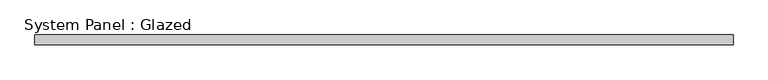
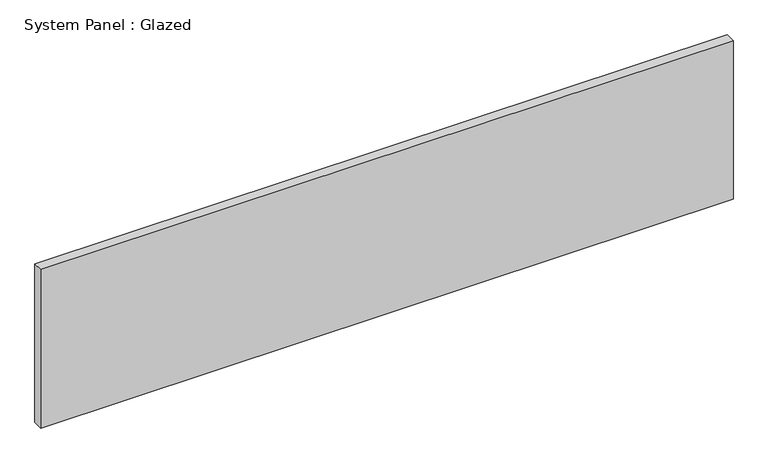
"""IFC4 building model written with IfcOpenShell, lengths in millimetres: plate geometry, System Panel : Glazed."""

import ifcopenshell
import ifcopenshell.guid

model = None  # the IFC model being written
_history = None  # IfcOwnerHistory: only IFC2X3 demands one
_inside = {}  # id of a spatial element -> (the spatial element, [elements in it])
_under = {}  # id of a project, library or spatial element -> (it, [spatial elements below it])
_declared = {}  # id of a project -> (the project, [libraries it declares])
_typed = {}  # id of a type object -> (the type object, [elements of that type])
_made_of = {}  # id of a material, layer set ... -> (it, [elements and type objects made of it])


def new_model(schema):
    """Start an empty IFC model of exactly this schema.

    Asked for "IFC4X3", IfcOpenShell would pick the latest addendum, in which some entities
    have other attributes; the version numbers below select the first issue.
    IFC2X3 requires an IfcOwnerHistory on every rooted entity: one is made here for all.
    """
    global model, _history
    if schema == "IFC4X3":
        model = ifcopenshell.file(schema_version=(4, 3, 0, 0))
    else:
        model = ifcopenshell.file(schema=schema)
    _inside.clear()
    _under.clear()
    _declared.clear()
    _typed.clear()
    _made_of.clear()
    _history = None
    if model.schema == "IFC2X3":
        org = make("IfcOrganization", Name="unknown")
        user = make(
            "IfcPersonAndOrganization",
            ThePerson=make("IfcPerson", FamilyName="unknown"),
            TheOrganization=org,
        )
        app = make(
            "IfcApplication",
            ApplicationDeveloper=org,
            Version="unknown",
            ApplicationFullName="unknown",
            ApplicationIdentifier="unknown",
        )
        _history = make(
            "IfcOwnerHistory",
            OwningUser=user,
            OwningApplication=app,
            ChangeAction="ADDED",
            CreationDate=0,
        )
    return model


def make(cls, **values):
    """One entity of the class cls with the attributes given. An attribute that is None is left unset."""
    return model.create_entity(
        cls, **{name: value for name, value in values.items() if value is not None}
    )


def rooted(cls, **values):
    """An entity with a GlobalId (a new one), such as an element, a storey or a relation."""
    return make(cls, GlobalId=ifcopenshell.guid.new(), OwnerHistory=_history, **values)


def si_unit(unit_type, name, prefix=None):
    """IfcSIUnit, for example si_unit("LENGTHUNIT", "METRE", prefix="MILLI")."""
    return make("IfcSIUnit", UnitType=unit_type, Prefix=prefix, Name=name)


def assignment(units):
    """IfcUnitAssignment: the units of a project."""
    return None if units is None else make("IfcUnitAssignment", Units=units)


def point(xyz):
    """IfcCartesianPoint."""
    return None if xyz is None else make("IfcCartesianPoint", Coordinates=xyz)


def direction(xyz):
    """IfcDirection."""
    return None if xyz is None else make("IfcDirection", DirectionRatios=xyz)


def frame(location, z_axis=None, x_axis=None):
    """IfcAxis2Placement3D, a coordinate frame: its origin and axes. An axis left out is left unset."""
    return make(
        "IfcAxis2Placement3D",
        Location=point(location),
        Axis=direction(z_axis),
        RefDirection=direction(x_axis),
    )


def origin():
    """The frame at (0, 0, 0) with its axes left unset."""
    return frame((0.0, 0.0, 0.0))


def origin_with_axes():
    """The frame at (0, 0, 0) with the z axis (0, 0, 1) and the x axis (1, 0, 0) written out."""
    return frame((0.0, 0.0, 0.0), z_axis=(0.0, 0.0, 1.0), x_axis=(1.0, 0.0, 0.0))


def place(relative_to, where):
    """IfcLocalPlacement: puts the frame where relative to a parent placement (None: the world)."""
    return make(
        "IfcLocalPlacement", PlacementRelTo=relative_to, RelativePlacement=where
    )


def context(
    kind, dimensions, precision=None, world=None, true_north=None, identifier=None
):
    """IfcGeometricRepresentationContext, for example the 3D "Model" context."""
    return make(
        "IfcGeometricRepresentationContext",
        ContextIdentifier=identifier,
        ContextType=kind,
        CoordinateSpaceDimension=dimensions,
        Precision=precision,
        WorldCoordinateSystem=world,
        TrueNorth=true_north,
    )


def project(units=None, contexts=None):
    """IfcProject with its units and contexts."""
    return rooted(
        "IfcProject",
        Name="project",
        RepresentationContexts=contexts,
        UnitsInContext=assignment(units),
    )


def spatial(cls, under=None, at=None, **own):
    """A site, building, storey or space (cls), placed at a placement, below another one or the project."""
    s = rooted(cls, ObjectPlacement=at, **own)
    if under is not None:
        _under.setdefault(under.id(), (under, []))[1].append(s)
    return s


def polyline(points):
    """IfcPolyline through the points."""
    return make("IfcPolyline", Points=[point(p) for p in points])


def outline(outer, holes=None, kind="AREA"):
    """IfcArbitraryClosedProfileDef: a profile drawn as a closed curve; with holes, ...WithVoids."""
    if holes is None:
        return make("IfcArbitraryClosedProfileDef", ProfileType=kind, OuterCurve=outer)
    return make(
        "IfcArbitraryProfileDefWithVoids",
        ProfileType=kind,
        OuterCurve=outer,
        InnerCurves=holes,
    )


def extrude(swept, where, along, depth):
    """IfcExtrudedAreaSolid: the profile swept, set in the frame where, extruded along a direction by depth."""
    return make(
        "IfcExtrudedAreaSolid",
        SweptArea=swept,
        Position=where,
        ExtrudedDirection=direction(along),
        Depth=depth,
    )


def shape(context_of_items, identifier, shape_type, items):
    """IfcShapeRepresentation: the items that make up one representation, for example the "Body"."""
    return make(
        "IfcShapeRepresentation",
        ContextOfItems=context_of_items,
        RepresentationIdentifier=identifier,
        RepresentationType=shape_type,
        Items=items,
    )


def source(mapping_origin, context_of_items, identifier, shape_type, items):
    """IfcRepresentationMap: a shape defined once, which mapped items show again and again."""
    return make(
        "IfcRepresentationMap",
        MappingOrigin=mapping_origin,
        MappedRepresentation=shape(context_of_items, identifier, shape_type, items),
    )


def transform(
    local_origin,
    x_axis=None,
    y_axis=None,
    z_axis=None,
    scale=None,
    scale2=None,
    scale3=None,
    uniform=True,
):
    """IfcCartesianTransformationOperator3D, or its non-uniform kind. x_axis, y_axis, z_axis: its Axis1, 2, 3."""
    if uniform:
        return make(
            "IfcCartesianTransformationOperator3D",
            Axis1=direction(x_axis),
            Axis2=direction(y_axis),
            LocalOrigin=point(local_origin),
            Scale=scale,
            Axis3=direction(z_axis),
        )
    return make(
        "IfcCartesianTransformationOperator3DnonUniform",
        Axis1=direction(x_axis),
        Axis2=direction(y_axis),
        LocalOrigin=point(local_origin),
        Scale=scale,
        Axis3=direction(z_axis),
        Scale2=scale2,
        Scale3=scale3,
    )


def mapped(mapping_source, mapping_target):
    """IfcMappedItem: shows the shape of a source again, moved by a transform."""
    return make(
        "IfcMappedItem", MappingSource=mapping_source, MappingTarget=mapping_target
    )


def made_of(thing, what):
    """Note that an element or type object is made of a material, layer set ...; save() writes the relation."""
    if what is not None:
        _made_of.setdefault(what.id(), (what, []))[1].append(thing)
    return thing


def element(
    cls,
    number,
    at=None,
    inside=None,
    cuts=None,
    type_object=None,
    material=None,
    context=None,
    identifier="Body",
    shape_type=None,
    held_by="IfcProductDefinitionShape",
    body=None,
    shapes=None,
    **own,
):
    """One element of the class cls, such as IfcWall. Its Tag is "e" and its number.

    at: its placement. inside: the storey or other place that contains it. cuts: it is an
    opening in that element (IfcRelVoidsElement). A single representation is given by context,
    identifier, shape_type and body (its items); several are given by shapes. held_by: the class
    of the entity that holds the representations. save() writes the other relations.
    """
    e = rooted(cls, Tag="e%d" % number, ObjectPlacement=at, **own)
    if body is not None:
        shapes = [shape(context, identifier, shape_type, body)]
    if shapes is not None:
        e.Representation = make(held_by, Representations=shapes)
    if inside is not None:
        _inside.setdefault(inside.id(), (inside, []))[1].append(e)
    if cuts is not None:
        rooted(
            "IfcRelVoidsElement", RelatingBuildingElement=cuts, RelatedOpeningElement=e
        )
    if type_object is not None:
        _typed.setdefault(type_object.id(), (type_object, []))[1].append(e)
    return made_of(e, material)


def aggregate(whole, parts):
    """IfcRelAggregates: a whole, such as a stair, and the parts it consists of."""
    return rooted("IfcRelAggregates", RelatingObject=whole, RelatedObjects=parts)


def save(model, path):
    """Write the relations noted so far, then the file.

    IfcRelAggregates (storeys below a building ...), IfcRelContainedInSpatialStructure (elements
    in a storey), IfcRelDefinesByType, IfcRelAssociatesMaterial and IfcRelDeclares: one each for
    every whole, place, type object, material and project.
    """
    for whole, parts in _under.values():
        aggregate(whole, parts)
    for where, things in _inside.values():
        rooted(
            "IfcRelContainedInSpatialStructure",
            RelatedElements=things,
            RelatingStructure=where,
        )
    for kind, things in _typed.values():
        rooted("IfcRelDefinesByType", RelatedObjects=things, RelatingType=kind)
    for what, things in _made_of.values():
        rooted("IfcRelAssociatesMaterial", RelatedObjects=things, RelatingMaterial=what)
    for by, libraries in _declared.values():
        rooted("IfcRelDeclares", RelatingContext=by, RelatedDefinitions=libraries)
    model.write(path)


def system_panel_glazed_66e2820e(model_context):
    return source(origin(), model_context, "Body", "SweptSolid", [
        extrude(outline(polyline([(877.5, -49.5), (-877.5, -49.5), (-877.5, -24.5), (877.5, -24.5), (877.5, -49.5)])), origin_with_axes(), (0.0, 0.0, 1.0), 425.0),
    ])


if __name__ == "__main__":
    model = new_model("IFC4")
    model_context = context("Model", 3, world=origin())
    ifc_project = project(units=[si_unit("LENGTHUNIT", "METRE", prefix="MILLI")], contexts=[model_context])
    site = spatial("IfcSite", under=ifc_project)
    building = spatial("IfcBuilding", under=site)
    placement = place(None, origin())
    system_panel_glazed_shape = system_panel_glazed_66e2820e(model_context)
    element("IfcPlate", 1, ObjectType="System Panel : Glazed", at=placement, inside=building, context=model_context, shape_type="MappedRepresentation", body=[
        mapped(system_panel_glazed_shape, transform((0.0, 0.0, 0.0), x_axis=(1.0, 0.0, 0.0), y_axis=(0.0, 1.0, 0.0), z_axis=(0.0, 0.0, 1.0))),
    ])
    save(model, "model.ifc")

# Revit data of these elements
# Type "System Panel : Glazed"
#   Keynote = "H11"
#   Construction Type Id = "GSP4R"
#   Analytic Construction = "1/8 in Pilkington single glazing"
#   Visual Light Transmittance = 0.9
#   Solar Heat Gain Coefficient = 0.86
#   Heat Transfer Coefficient (U) = 6.7069 W/(m²·K)
# Element 1 (IfcPlate, "System Panel : Glazed")
#   Materials on its faces: "Glass"
# Materials
#   "Glass": class "Glass", colour RGB 0 128 192, transparency 0.9, Description = "Soda Lime Glass", Cost = 0
